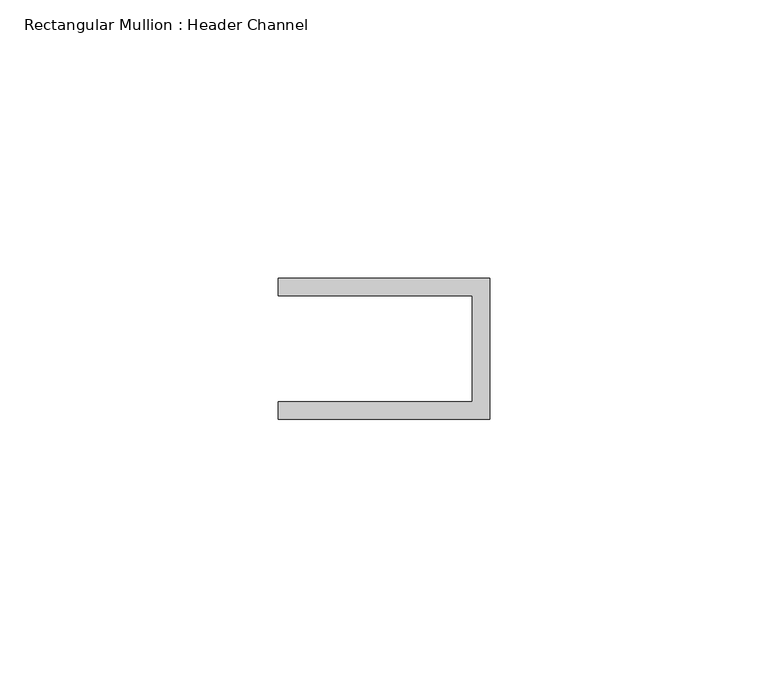
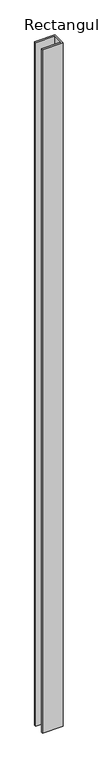
"""IFC4 building model written with IfcOpenShell, lengths in millimetres: member geometry, Rectangular Mullion : Header Channel."""

import ifcopenshell
import ifcopenshell.guid

model = None  # the IFC model being written
_history = None  # IfcOwnerHistory: only IFC2X3 demands one
_inside = {}  # id of a spatial element -> (the spatial element, [elements in it])
_under = {}  # id of a project, library or spatial element -> (it, [spatial elements below it])
_declared = {}  # id of a project -> (the project, [libraries it declares])
_typed = {}  # id of a type object -> (the type object, [elements of that type])
_made_of = {}  # id of a material, layer set ... -> (it, [elements and type objects made of it])


def new_model(schema):
    """Start an empty IFC model of exactly this schema.

    Asked for "IFC4X3", IfcOpenShell would pick the latest addendum, in which some entities
    have other attributes; the version numbers below select the first issue.
    IFC2X3 requires an IfcOwnerHistory on every rooted entity: one is made here for all.
    """
    global model, _history
    if schema == "IFC4X3":
        model = ifcopenshell.file(schema_version=(4, 3, 0, 0))
    else:
        model = ifcopenshell.file(schema=schema)
    _inside.clear()
    _under.clear()
    _declared.clear()
    _typed.clear()
    _made_of.clear()
    _history = None
    if model.schema == "IFC2X3":
        org = make("IfcOrganization", Name="unknown")
        user = make(
            "IfcPersonAndOrganization",
            ThePerson=make("IfcPerson", FamilyName="unknown"),
            TheOrganization=org,
        )
        app = make(
            "IfcApplication",
            ApplicationDeveloper=org,
            Version="unknown",
            ApplicationFullName="unknown",
            ApplicationIdentifier="unknown",
        )
        _history = make(
            "IfcOwnerHistory",
            OwningUser=user,
            OwningApplication=app,
            ChangeAction="ADDED",
            CreationDate=0,
        )
    return model


def make(cls, **values):
    """One entity of the class cls with the attributes given. An attribute that is None is left unset."""
    return model.create_entity(
        cls, **{name: value for name, value in values.items() if value is not None}
    )


def rooted(cls, **values):
    """An entity with a GlobalId (a new one), such as an element, a storey or a relation."""
    return make(cls, GlobalId=ifcopenshell.guid.new(), OwnerHistory=_history, **values)


def si_unit(unit_type, name, prefix=None):
    """IfcSIUnit, for example si_unit("LENGTHUNIT", "METRE", prefix="MILLI")."""
    return make("IfcSIUnit", UnitType=unit_type, Prefix=prefix, Name=name)


def assignment(units):
    """IfcUnitAssignment: the units of a project."""
    return None if units is None else make("IfcUnitAssignment", Units=units)


def point(xyz):
    """IfcCartesianPoint."""
    return None if xyz is None else make("IfcCartesianPoint", Coordinates=xyz)


def direction(xyz):
    """IfcDirection."""
    return None if xyz is None else make("IfcDirection", DirectionRatios=xyz)


def frame(location, z_axis=None, x_axis=None):
    """IfcAxis2Placement3D, a coordinate frame: its origin and axes. An axis left out is left unset."""
    return make(
        "IfcAxis2Placement3D",
        Location=point(location),
        Axis=direction(z_axis),
        RefDirection=direction(x_axis),
    )


def origin():
    """The frame at (0, 0, 0) with its axes left unset."""
    return frame((0.0, 0.0, 0.0))


def place(relative_to, where):
    """IfcLocalPlacement: puts the frame where relative to a parent placement (None: the world)."""
    return make(
        "IfcLocalPlacement", PlacementRelTo=relative_to, RelativePlacement=where
    )


def context(
    kind, dimensions, precision=None, world=None, true_north=None, identifier=None
):
    """IfcGeometricRepresentationContext, for example the 3D "Model" context."""
    return make(
        "IfcGeometricRepresentationContext",
        ContextIdentifier=identifier,
        ContextType=kind,
        CoordinateSpaceDimension=dimensions,
        Precision=precision,
        WorldCoordinateSystem=world,
        TrueNorth=true_north,
    )


def project(units=None, contexts=None):
    """IfcProject with its units and contexts."""
    return rooted(
        "IfcProject",
        Name="project",
        RepresentationContexts=contexts,
        UnitsInContext=assignment(units),
    )


def spatial(cls, under=None, at=None, **own):
    """A site, building, storey or space (cls), placed at a placement, below another one or the project."""
    s = rooted(cls, ObjectPlacement=at, **own)
    if under is not None:
        _under.setdefault(under.id(), (under, []))[1].append(s)
    return s


def polyline(points):
    """IfcPolyline through the points."""
    return make("IfcPolyline", Points=[point(p) for p in points])


def outline(outer, holes=None, kind="AREA"):
    """IfcArbitraryClosedProfileDef: a profile drawn as a closed curve; with holes, ...WithVoids."""
    if holes is None:
        return make("IfcArbitraryClosedProfileDef", ProfileType=kind, OuterCurve=outer)
    return make(
        "IfcArbitraryProfileDefWithVoids",
        ProfileType=kind,
        OuterCurve=outer,
        InnerCurves=holes,
    )


def extrude(swept, where, along, depth):
    """IfcExtrudedAreaSolid: the profile swept, set in the frame where, extruded along a direction by depth."""
    return make(
        "IfcExtrudedAreaSolid",
        SweptArea=swept,
        Position=where,
        ExtrudedDirection=direction(along),
        Depth=depth,
    )


def shape(context_of_items, identifier, shape_type, items):
    """IfcShapeRepresentation: the items that make up one representation, for example the "Body"."""
    return make(
        "IfcShapeRepresentation",
        ContextOfItems=context_of_items,
        RepresentationIdentifier=identifier,
        RepresentationType=shape_type,
        Items=items,
    )


def source(mapping_origin, context_of_items, identifier, shape_type, items):
    """IfcRepresentationMap: a shape defined once, which mapped items show again and again."""
    return make(
        "IfcRepresentationMap",
        MappingOrigin=mapping_origin,
        MappedRepresentation=shape(context_of_items, identifier, shape_type, items),
    )


def transform(
    local_origin,
    x_axis=None,
    y_axis=None,
    z_axis=None,
    scale=None,
    scale2=None,
    scale3=None,
    uniform=True,
):
    """IfcCartesianTransformationOperator3D, or its non-uniform kind. x_axis, y_axis, z_axis: its Axis1, 2, 3."""
    if uniform:
        return make(
            "IfcCartesianTransformationOperator3D",
            Axis1=direction(x_axis),
            Axis2=direction(y_axis),
            LocalOrigin=point(local_origin),
            Scale=scale,
            Axis3=direction(z_axis),
        )
    return make(
        "IfcCartesianTransformationOperator3DnonUniform",
        Axis1=direction(x_axis),
        Axis2=direction(y_axis),
        LocalOrigin=point(local_origin),
        Scale=scale,
        Axis3=direction(z_axis),
        Scale2=scale2,
        Scale3=scale3,
    )


def mapped(mapping_source, mapping_target):
    """IfcMappedItem: shows the shape of a source again, moved by a transform."""
    return make(
        "IfcMappedItem", MappingSource=mapping_source, MappingTarget=mapping_target
    )


def made_of(thing, what):
    """Note that an element or type object is made of a material, layer set ...; save() writes the relation."""
    if what is not None:
        _made_of.setdefault(what.id(), (what, []))[1].append(thing)
    return thing


def element(
    cls,
    number,
    at=None,
    inside=None,
    cuts=None,
    type_object=None,
    material=None,
    context=None,
    identifier="Body",
    shape_type=None,
    held_by="IfcProductDefinitionShape",
    body=None,
    shapes=None,
    **own,
):
    """One element of the class cls, such as IfcWall. Its Tag is "e" and its number.

    at: its placement. inside: the storey or other place that contains it. cuts: it is an
    opening in that element (IfcRelVoidsElement). A single representation is given by context,
    identifier, shape_type and body (its items); several are given by shapes. held_by: the class
    of the entity that holds the representations. save() writes the other relations.
    """
    e = rooted(cls, Tag="e%d" % number, ObjectPlacement=at, **own)
    if body is not None:
        shapes = [shape(context, identifier, shape_type, body)]
    if shapes is not None:
        e.Representation = make(held_by, Representations=shapes)
    if inside is not None:
        _inside.setdefault(inside.id(), (inside, []))[1].append(e)
    if cuts is not None:
        rooted(
            "IfcRelVoidsElement", RelatingBuildingElement=cuts, RelatedOpeningElement=e
        )
    if type_object is not None:
        _typed.setdefault(type_object.id(), (type_object, []))[1].append(e)
    return made_of(e, material)


def aggregate(whole, parts):
    """IfcRelAggregates: a whole, such as a stair, and the parts it consists of."""
    return rooted("IfcRelAggregates", RelatingObject=whole, RelatedObjects=parts)


def save(model, path):
    """Write the relations noted so far, then the file.

    IfcRelAggregates (storeys below a building ...), IfcRelContainedInSpatialStructure (elements
    in a storey), IfcRelDefinesByType, IfcRelAssociatesMaterial and IfcRelDeclares: one each for
    every whole, place, type object, material and project.
    """
    for whole, parts in _under.values():
        aggregate(whole, parts)
    for where, things in _inside.values():
        rooted(
            "IfcRelContainedInSpatialStructure",
            RelatedElements=things,
            RelatingStructure=where,
        )
    for kind, things in _typed.values():
        rooted("IfcRelDefinesByType", RelatedObjects=things, RelatingType=kind)
    for what, things in _made_of.values():
        rooted("IfcRelAssociatesMaterial", RelatedObjects=things, RelatingMaterial=what)
    for by, libraries in _declared.values():
        rooted("IfcRelDeclares", RelatingContext=by, RelatedDefinitions=libraries)
    model.write(path)


def rectangular_mullion_header_channel_7ecd0432(model_context):
    return source(origin(), model_context, "Body", "SweptSolid", [
        extrude(outline(polyline([(0.0, 12.7), (0.0, -12.7), (-38.1, -12.7), (-38.1, -9.525), (-3.175, -9.525), (-3.175, 9.525), (-38.1, 9.525), (-38.1, 12.7), (0.0, 12.7)])), frame((0.0, 0.0, -1346.2), z_axis=(0.0, 0.0, 1.0), x_axis=(1.0, 0.0, 0.0)), (0.0, 0.0, 1.0), 1346.2),
    ])


if __name__ == "__main__":
    model = new_model("IFC4")
    model_context = context("Model", 3, world=origin())
    ifc_project = project(units=[si_unit("LENGTHUNIT", "METRE", prefix="MILLI")], contexts=[model_context])
    site = spatial("IfcSite", under=ifc_project)
    building = spatial("IfcBuilding", under=site)
    placement = place(None, origin())
    rectangular_mullion_header_channel_shape = rectangular_mullion_header_channel_7ecd0432(model_context)
    element("IfcMember", 1, ObjectType="Rectangular Mullion : Header Channel", at=placement, inside=building, context=model_context, shape_type="MappedRepresentation", body=[
        mapped(rectangular_mullion_header_channel_shape, transform((0.0, 0.0, 0.0), x_axis=(1.0, 0.0, 0.0), y_axis=(0.0, 1.0, 0.0), z_axis=(0.0, 0.0, 1.0))),
    ])
    save(model, "model.ifc")

# Revit data of these elements
# Type "Rectangular Mullion : Header Channel"
#   built-in parameter 1007322 = 0.0833333 (stored number, unit not read)
#   built-in parameter 1007321 = -0.03125 (stored number, unit not read)
#   built-in parameter 1007320 = 0.0416667 (stored number, unit not read)
# Element 1 (IfcMember, "Rectangular Mullion : Header Channel")
#   Materials on its faces: "ALUM"
# Materials
#   "ALUM": class "Generic", colour RGB 157 157 157, transparency 0, Cost = 0
